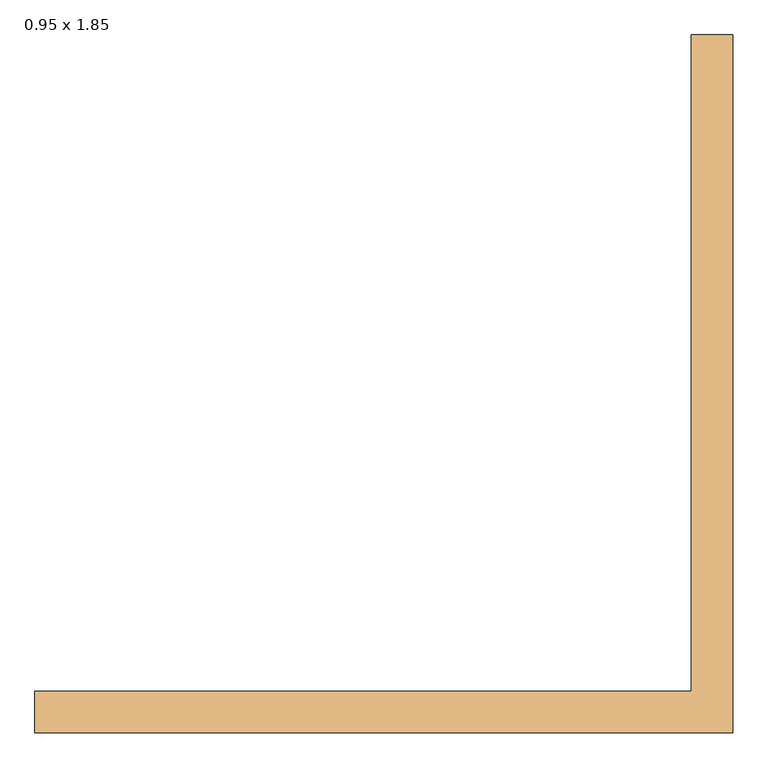
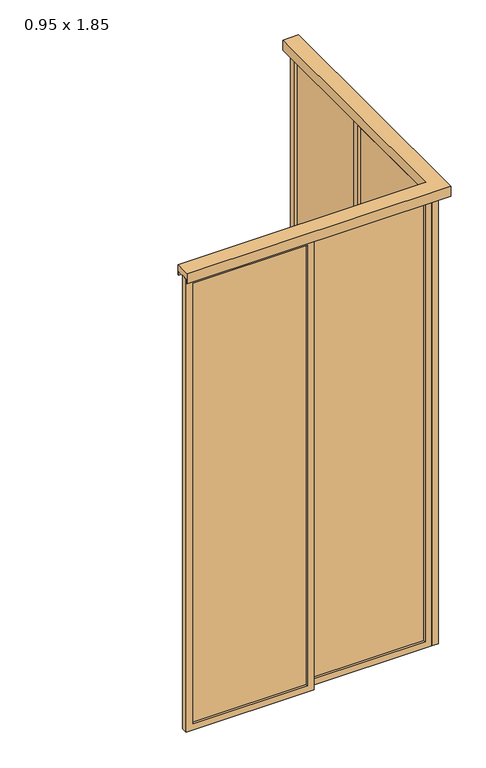
"""IFC4 building model written with IfcOpenShell, lengths in millimetres: door geometry, CC_ND-200_BOX-L-BANHEIRO : 0.95 x 1.85."""

from ifc_helpers import new_model, si_unit, frame, origin, origin_with_axes, place, context, project, spatial, polyline, outline, extrude, faceted_brep, source, transform, mapped, element, save


def door_0_95_x_1_85_64086e03(model_context):
    return source(origin(), model_context, "Body", "SolidModel", [
        extrude(outline(polyline([(975.0, 50.0), (975.0, 25.0), (950.0, 25.0), (950.0, 50.0), (975.0, 50.0)])), origin_with_axes(), (0.0, 0.0, 1.0), 1825.0),
        extrude(outline(polyline([(965.0, 527.5), (965.0, 60.0), (960.0, 60.0), (960.0, 527.5), (965.0, 527.5)])), frame((0.0, 0.0, 10.0), z_axis=(0.0, 0.0, 1.0), x_axis=(1.0, 0.0, 0.0)), (0.0, 0.0, 1.0), 1805.0),
        faceted_brep([(975.0, 512.5, 1800.0), (965.0, 512.5, 1800.0), (965.0, 512.5, 25.0), (975.0, 512.5, 25.0), (965.0, 527.5, 1815.0), (965.0, 527.5, 10.0), (965.0, 60.0, 10.0), (965.0, 60.0, 1815.0), (965.0, 75.0, 1800.0), (965.0, 75.0, 25.0), (975.0, 75.0, 25.0), (975.0, 50.0, 1825.0), (975.0, 50.0, 0.0), (975.0, 537.5, 0.0), (975.0, 537.5, 1825.0), (975.0, 75.0, 1800.0), (950.0, 537.5, 1825.0), (950.0, 537.5, 0.0), (950.0, 50.0, 0.0), (950.0, 50.0, 1825.0), (950.0, 75.0, 1800.0), (950.0, 75.0, 25.0), (950.0, 512.5, 25.0), (950.0, 512.5, 1800.0), (960.0, 75.0, 25.0), (960.0, 75.0, 1800.0), (960.0, 512.5, 25.0), (960.0, 512.5, 1800.0), (960.0, 527.5, 1815.0), (960.0, 527.5, 10.0), (960.0, 60.0, 1815.0), (960.0, 60.0, 10.0)], [[[0, 1, 2, 3]], [[4, 5, 6, 7], [8, 9, 2, 1]], [[3, 2, 9, 10]], [[11, 12, 13, 14], [0, 3, 10, 15]], [[16, 14, 13, 17]], [[17, 13, 12, 18]], [[16, 17, 18, 19], [20, 21, 22, 23]], [[10, 9, 8, 15]], [[18, 12, 11, 19]], [[24, 21, 20, 25]], [[26, 22, 21, 24]], [[27, 23, 22, 26]], [[4, 28, 29, 5]], [[30, 31, 29, 28], [27, 26, 24, 25]], [[5, 29, 31, 6]], [[6, 31, 30, 7]], [[15, 8, 1, 0]], [[19, 11, 14, 16]], [[7, 30, 28, 4]], [[25, 20, 23, 27]]]),
        extrude(outline(polyline([(990.0, 990.0), (990.0, 522.5), (985.0, 522.5), (985.0, 990.0), (990.0, 990.0)])), frame((0.0, 0.0, 10.0), z_axis=(0.0, 0.0, 1.0), x_axis=(1.0, 0.0, 0.0)), (0.0, 0.0, 1.0), 1805.0),
        faceted_brep([(1000.0, 975.0, 1800.0), (990.0, 975.0, 1800.0), (990.0, 975.0, 25.0), (1000.0, 975.0, 25.0), (990.0, 990.0, 1815.0), (990.0, 990.0, 10.0), (990.0, 522.5, 10.0), (990.0, 522.5, 1815.0), (990.0, 537.5, 1800.0), (990.0, 537.5, 25.0), (1000.0, 537.5, 25.0), (1000.0, 512.5, 1825.0), (1000.0, 512.5, 0.0), (1000.0, 1000.0, 0.0), (1000.0, 1000.0, 1825.0), (1000.0, 537.5, 1800.0), (975.0, 1000.0, 1825.0), (975.0, 1000.0, 0.0), (975.0, 512.5, 0.0), (975.0, 512.5, 1825.0), (975.0, 537.5, 1800.0), (975.0, 537.5, 25.0), (975.0, 975.0, 25.0), (975.0, 975.0, 1800.0), (985.0, 537.5, 25.0), (985.0, 537.5, 1800.0), (985.0, 975.0, 25.0), (985.0, 975.0, 1800.0), (985.0, 990.0, 1815.0), (985.0, 990.0, 10.0), (985.0, 522.5, 1815.0), (985.0, 522.5, 10.0)], [[[0, 1, 2, 3]], [[4, 5, 6, 7], [8, 9, 2, 1]], [[3, 2, 9, 10]], [[11, 12, 13, 14], [0, 3, 10, 15]], [[16, 14, 13, 17]], [[17, 13, 12, 18]], [[16, 17, 18, 19], [20, 21, 22, 23]], [[10, 9, 8, 15]], [[18, 12, 11, 19]], [[24, 21, 20, 25]], [[26, 22, 21, 24]], [[27, 23, 22, 26]], [[4, 28, 29, 5]], [[30, 31, 29, 28], [27, 26, 24, 25]], [[5, 29, 31, 6]], [[6, 31, 30, 7]], [[15, 8, 1, 0]], [[19, 11, 14, 16]], [[7, 30, 28, 4]], [[25, 20, 23, 27]]]),
        extrude(outline(polyline([(477.5, 15.0), (477.5, 10.0), (10.0, 10.0), (10.0, 15.0), (477.5, 15.0)])), frame((0.0, 0.0, 10.0), z_axis=(0.0, 0.0, 1.0), x_axis=(1.0, 0.0, 0.0)), (0.0, 0.0, 1.0), 1805.0),
        faceted_brep([(462.5, 15.0, 1800.0), (462.5, 25.0, 1800.0), (462.5, 25.0, 25.0), (462.5, 15.0, 25.0), (487.5, 25.0, 1825.0), (487.5, 25.0, 0.0), (0.0, 25.0, 0.0), (0.0, 25.0, 1825.0), (25.0, 25.0, 1800.0), (25.0, 25.0, 25.0), (25.0, 15.0, 25.0), (10.0, 15.0, 1815.0), (10.0, 15.0, 10.0), (477.5, 15.0, 10.0), (477.5, 15.0, 1815.0), (25.0, 15.0, 1800.0), (487.5, 0.0, 1825.0), (487.5, 0.0, 0.0), (0.0, 0.0, 1825.0), (0.0, 0.0, 0.0), (462.5, 0.0, 1800.0), (462.5, 0.0, 25.0), (25.0, 0.0, 25.0), (25.0, 0.0, 1800.0), (462.5, 10.0, 1800.0), (462.5, 10.0, 25.0), (25.0, 10.0, 25.0), (25.0, 10.0, 1800.0), (477.5, 10.0, 1815.0), (477.5, 10.0, 10.0), (10.0, 10.0, 10.0), (10.0, 10.0, 1815.0)], [[[0, 1, 2, 3]], [[4, 5, 6, 7], [8, 9, 2, 1]], [[3, 2, 9, 10]], [[11, 12, 13, 14], [0, 3, 10, 15]], [[4, 16, 17, 5]], [[18, 19, 17, 16], [20, 21, 22, 23]], [[5, 17, 19, 6]], [[10, 9, 8, 15]], [[6, 19, 18, 7]], [[20, 24, 25, 21]], [[21, 25, 26, 22]], [[22, 26, 27, 23]], [[28, 14, 13, 29]], [[29, 13, 12, 30]], [[28, 29, 30, 31], [27, 26, 25, 24]], [[30, 12, 11, 31]], [[15, 8, 1, 0]], [[7, 18, 16, 4]], [[31, 11, 14, 28]], [[23, 27, 24, 20]]]),
        extrude(outline(polyline([(940.0, 40.0), (940.0, 35.0), (472.5, 35.0), (472.5, 40.0), (940.0, 40.0)])), frame((0.0, 0.0, 10.0), z_axis=(0.0, 0.0, 1.0), x_axis=(1.0, 0.0, 0.0)), (0.0, 0.0, 1.0), 1805.0),
        faceted_brep([(925.0, 40.0, 1800.0), (925.0, 50.0, 1800.0), (925.0, 50.0, 25.0), (925.0, 40.0, 25.0), (950.0, 50.0, 1825.0), (950.0, 50.0, 0.0), (462.5, 50.0, 0.0), (462.5, 50.0, 1825.0), (487.5, 50.0, 1800.0), (487.5, 50.0, 25.0), (487.5, 40.0, 25.0), (472.5, 40.0, 1815.0), (472.5, 40.0, 10.0), (940.0, 40.0, 10.0), (940.0, 40.0, 1815.0), (487.5, 40.0, 1800.0), (950.0, 25.0, 1825.0), (950.0, 25.0, 0.0), (462.5, 25.0, 1825.0), (462.5, 25.0, 0.0), (925.0, 25.0, 1800.0), (925.0, 25.0, 25.0), (487.5, 25.0, 25.0), (487.5, 25.0, 1800.0), (925.0, 35.0, 1800.0), (925.0, 35.0, 25.0), (487.5, 35.0, 25.0), (487.5, 35.0, 1800.0), (940.0, 35.0, 1815.0), (940.0, 35.0, 10.0), (472.5, 35.0, 10.0), (472.5, 35.0, 1815.0)], [[[0, 1, 2, 3]], [[4, 5, 6, 7], [8, 9, 2, 1]], [[3, 2, 9, 10]], [[11, 12, 13, 14], [0, 3, 10, 15]], [[4, 16, 17, 5]], [[18, 19, 17, 16], [20, 21, 22, 23]], [[5, 17, 19, 6]], [[10, 9, 8, 15]], [[6, 19, 18, 7]], [[20, 24, 25, 21]], [[21, 25, 26, 22]], [[22, 26, 27, 23]], [[28, 14, 13, 29]], [[29, 13, 12, 30]], [[28, 29, 30, 31], [27, 26, 25, 24]], [[30, 12, 11, 31]], [[15, 8, 1, 0]], [[7, 18, 16, 4]], [[31, 11, 14, 28]], [[23, 27, 24, 20]]]),
        faceted_brep([(0.0, -5.0, 1810.0), (0.0, -5.0, 1850.0), (0.0, 55.0, 1850.0), (0.0, 55.0, 1810.0), (0.0, 50.0, 1810.0), (0.0, 50.0, 1825.0), (0.0, 0.0, 1825.0), (0.0, 0.0, 1810.0), (1005.0, 1000.0, 1810.0), (1000.0, 1000.0, 1810.0), (1000.0, 1000.0, 1825.0), (950.0, 1000.0, 1825.0), (950.0, 1000.0, 1810.0), (945.0, 1000.0, 1810.0), (945.0, 1000.0, 1850.0), (1005.0, 1000.0, 1850.0), (1005.0, -5.0, 1810.0), (1005.0, -5.0, 1850.0), (945.0, 55.0, 1850.0), (945.0, 55.0, 1810.0), (950.0, 50.0, 1810.0), (950.0, 50.0, 1825.0), (1000.0, 0.0, 1825.0), (1000.0, 0.0, 1810.0)], [[[0, 1, 2, 3, 4, 5, 6, 7]], [[8, 9, 10, 11, 12, 13, 14, 15]], [[1, 0, 16, 17]], [[2, 1, 17, 15, 14, 18]], [[3, 2, 18, 19]], [[4, 3, 19, 13, 12, 20]], [[5, 4, 20, 21]], [[6, 5, 21, 11, 10, 22]], [[7, 6, 22, 23]], [[0, 7, 23, 9, 8, 16]], [[17, 16, 8, 15]], [[19, 18, 14, 13]], [[21, 20, 12, 11]], [[23, 22, 10, 9]]]),
    ])


if __name__ == "__main__":
    model = new_model("IFC4")
    model_context = context("Model", 3, world=origin())
    ifc_project = project(units=[si_unit("LENGTHUNIT", "METRE", prefix="MILLI")], contexts=[model_context])
    site = spatial("IfcSite", under=ifc_project)
    building = spatial("IfcBuilding", under=site)
    placement = place(None, origin())
    door_0_95_x_1_85_shape = door_0_95_x_1_85_64086e03(model_context)
    element("IfcDoor", 1, ObjectType="CC_ND-200_BOX-L-BANHEIRO : 0.95 x 1.85", at=placement, inside=building, context=model_context, shape_type="MappedRepresentation", body=[
        mapped(door_0_95_x_1_85_shape, transform((0.0, 0.0, 0.0), x_axis=(1.0, 0.0, 0.0), y_axis=(0.0, 1.0, 0.0), z_axis=(0.0, 0.0, 1.0))),
    ])
    save(model, "model.ifc")

# Revit data of these elements
# Type "CC_ND-200_BOX-L-BANHEIRO : 0.95 x 1.85"
#   Type Mark = "144"
#   Width = 0.95 m
#   Material montante = Aluminio
#   Materia vidro = Vidro
# Element 1 (IfcDoor, "CC_ND-200_BOX-L-BANHEIRO : 0.95 x 1.85")
#   Materials on its faces: "Aluminio", "Vidro"
# Materials
#   "Aluminio": class "Genérico", colour RGB 120 120 120, transparency 0, Cost = 0
#   "Vidro": class "Vidro", colour RGB 230 230 230, transparency 0.75, Description = "JANELA COM 04 FOLHAS DE CORRER E VIDRO TRANSPARENTE 6mm", Cost = 0
